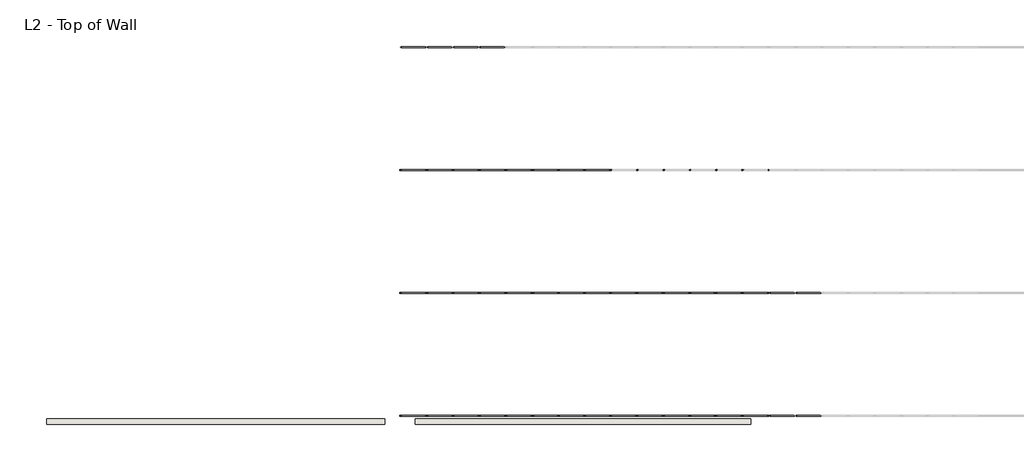
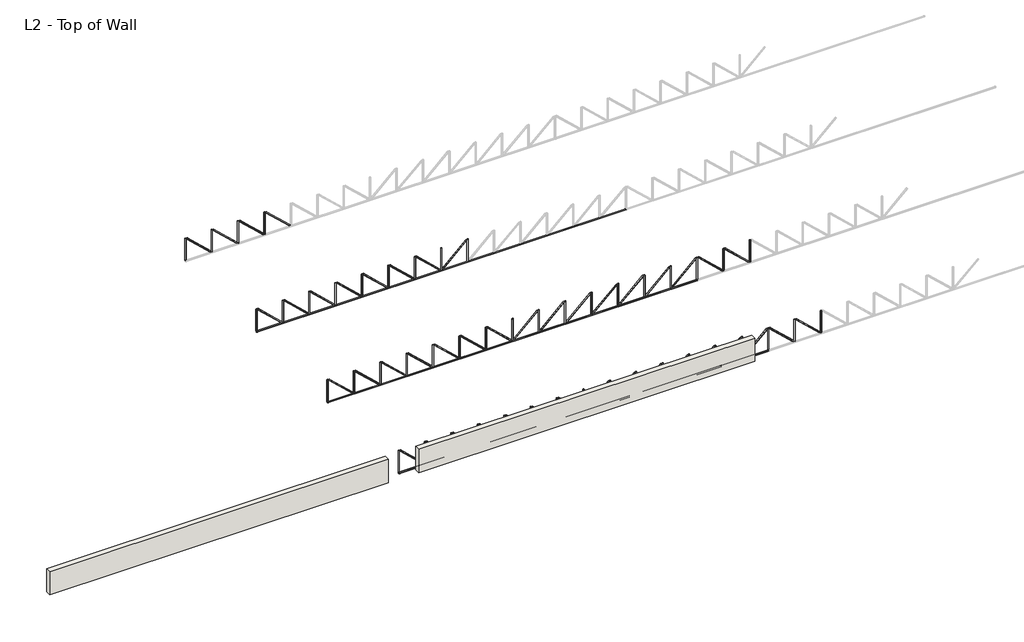
# One storey, part 1 of 4: 96 beams, 2 walls.
"""IFC4 building model written with IfcOpenShell, lengths in millimetres."""

import ifcopenshell
import ifcopenshell.guid

model = None  # the IFC model being written
_history = None  # IfcOwnerHistory: only IFC2X3 demands one
_inside = {}  # id of a spatial element -> (the spatial element, [elements in it])
_under = {}  # id of a project, library or spatial element -> (it, [spatial elements below it])
_declared = {}  # id of a project -> (the project, [libraries it declares])
_typed = {}  # id of a type object -> (the type object, [elements of that type])
_made_of = {}  # id of a material, layer set ... -> (it, [elements and type objects made of it])


def new_model(schema):
    """Start an empty IFC model of exactly this schema.

    Asked for "IFC4X3", IfcOpenShell would pick the latest addendum, in which some entities
    have other attributes; the version numbers below select the first issue.
    IFC2X3 requires an IfcOwnerHistory on every rooted entity: one is made here for all.
    """
    global model, _history
    if schema == "IFC4X3":
        model = ifcopenshell.file(schema_version=(4, 3, 0, 0))
    else:
        model = ifcopenshell.file(schema=schema)
    _inside.clear()
    _under.clear()
    _declared.clear()
    _typed.clear()
    _made_of.clear()
    _history = None
    if model.schema == "IFC2X3":
        org = make("IfcOrganization", Name="unknown")
        user = make(
            "IfcPersonAndOrganization",
            ThePerson=make("IfcPerson", FamilyName="unknown"),
            TheOrganization=org,
        )
        app = make(
            "IfcApplication",
            ApplicationDeveloper=org,
            Version="unknown",
            ApplicationFullName="unknown",
            ApplicationIdentifier="unknown",
        )
        _history = make(
            "IfcOwnerHistory",
            OwningUser=user,
            OwningApplication=app,
            ChangeAction="ADDED",
            CreationDate=0,
        )
    return model


def make(cls, **values):
    """One entity of the class cls with the attributes given. An attribute that is None is left unset."""
    return model.create_entity(
        cls, **{name: value for name, value in values.items() if value is not None}
    )


def rooted(cls, **values):
    """An entity with a GlobalId (a new one), such as an element, a storey or a relation."""
    return make(cls, GlobalId=ifcopenshell.guid.new(), OwnerHistory=_history, **values)


def si_unit(unit_type, name, prefix=None):
    """IfcSIUnit, for example si_unit("LENGTHUNIT", "METRE", prefix="MILLI")."""
    return make("IfcSIUnit", UnitType=unit_type, Prefix=prefix, Name=name)


def assignment(units):
    """IfcUnitAssignment: the units of a project."""
    return None if units is None else make("IfcUnitAssignment", Units=units)


def point(xyz):
    """IfcCartesianPoint."""
    return None if xyz is None else make("IfcCartesianPoint", Coordinates=xyz)


def direction(xyz):
    """IfcDirection."""
    return None if xyz is None else make("IfcDirection", DirectionRatios=xyz)


def frame(location, z_axis=None, x_axis=None):
    """IfcAxis2Placement3D, a coordinate frame: its origin and axes. An axis left out is left unset."""
    return make(
        "IfcAxis2Placement3D",
        Location=point(location),
        Axis=direction(z_axis),
        RefDirection=direction(x_axis),
    )


def frame_2d(location, x_axis=None):
    """IfcAxis2Placement2D, a coordinate frame in the plane: its origin and x axis."""
    return make(
        "IfcAxis2Placement2D", Location=point(location), RefDirection=direction(x_axis)
    )


def origin():
    """The frame at (0, 0, 0) with its axes left unset."""
    return frame((0.0, 0.0, 0.0))


def origin_2d():
    """The frame at (0, 0) in the plane with its x axis left unset."""
    return frame_2d((0.0, 0.0))


def place(relative_to, where):
    """IfcLocalPlacement: puts the frame where relative to a parent placement (None: the world)."""
    return make(
        "IfcLocalPlacement", PlacementRelTo=relative_to, RelativePlacement=where
    )


def context(
    kind, dimensions, precision=None, world=None, true_north=None, identifier=None
):
    """IfcGeometricRepresentationContext, for example the 3D "Model" context."""
    return make(
        "IfcGeometricRepresentationContext",
        ContextIdentifier=identifier,
        ContextType=kind,
        CoordinateSpaceDimension=dimensions,
        Precision=precision,
        WorldCoordinateSystem=world,
        TrueNorth=true_north,
    )


def project(units=None, contexts=None):
    """IfcProject with its units and contexts."""
    return rooted(
        "IfcProject",
        Name="project",
        RepresentationContexts=contexts,
        UnitsInContext=assignment(units),
    )


def spatial(cls, under=None, at=None, **own):
    """A site, building, storey or space (cls), placed at a placement, below another one or the project."""
    s = rooted(cls, ObjectPlacement=at, **own)
    if under is not None:
        _under.setdefault(under.id(), (under, []))[1].append(s)
    return s


def circle_curve(where, radius):
    """IfcCircle in the frame where."""
    return make("IfcCircle", Position=where, Radius=radius)


def trimmed(basis, trim1, trim2, sense, master):
    """IfcTrimmedCurve: the piece of a basis curve between two trims."""
    return make(
        "IfcTrimmedCurve",
        BasisCurve=basis,
        Trim1=trim1,
        Trim2=trim2,
        SenseAgreement=sense,
        MasterRepresentation=master,
    )


def segment(curve, same_sense, transition):
    """IfcCompositeCurveSegment."""
    return make(
        "IfcCompositeCurveSegment",
        Transition=transition,
        SameSense=same_sense,
        ParentCurve=curve,
    )


def composite_curve(segments, self_intersect=None):
    """IfcCompositeCurve: segments joined end to end."""
    return make("IfcCompositeCurve", Segments=segments, SelfIntersect=self_intersect)


def outline(outer, holes=None, kind="AREA"):
    """IfcArbitraryClosedProfileDef: a profile drawn as a closed curve; with holes, ...WithVoids."""
    if holes is None:
        return make("IfcArbitraryClosedProfileDef", ProfileType=kind, OuterCurve=outer)
    return make(
        "IfcArbitraryProfileDefWithVoids",
        ProfileType=kind,
        OuterCurve=outer,
        InnerCurves=holes,
    )


def extrude(swept, where, along, depth):
    """IfcExtrudedAreaSolid: the profile swept, set in the frame where, extruded along a direction by depth."""
    return make(
        "IfcExtrudedAreaSolid",
        SweptArea=swept,
        Position=where,
        ExtrudedDirection=direction(along),
        Depth=depth,
    )


def faces_of(points, faces, orient=None, outer=None):
    """IfcFace entities. A face is a list of loops; a loop is a list of indices into points, from 0.

    orient and outer hold one flag for each loop. By default every Orientation is true, the
    first loop of a face is its IfcFaceOuterBound and the others are IfcFaceBound.
    """
    made = []
    for i, loops in enumerate(faces):
        bounds = []
        for j, loop in enumerate(loops):
            is_outer = j == 0 if outer is None else outer[i][j]
            bounds.append(
                make(
                    "IfcFaceOuterBound" if is_outer else "IfcFaceBound",
                    Bound=make("IfcPolyLoop", Polygon=[points[k] for k in loop]),
                    Orientation=True if orient is None else orient[i][j],
                )
            )
        made.append(make("IfcFace", Bounds=bounds))
    return made


def faceted_brep(points, faces, orient=None, outer=None, voids=None):
    """IfcFacetedBrep: a solid bounded by flat faces; with voids (closed shells), ...WithVoids."""
    shared = [point(p) for p in points]
    hull = make("IfcClosedShell", CfsFaces=faces_of(shared, faces, orient, outer))
    if voids is None:
        return make("IfcFacetedBrep", Outer=hull)
    return make(
        "IfcFacetedBrepWithVoids",
        Outer=hull,
        Voids=[
            make(cls, CfsFaces=faces_of(shared, fs, o, b)) for cls, fs, o, b in voids
        ],
    )


def shape(context_of_items, identifier, shape_type, items):
    """IfcShapeRepresentation: the items that make up one representation, for example the "Body"."""
    return make(
        "IfcShapeRepresentation",
        ContextOfItems=context_of_items,
        RepresentationIdentifier=identifier,
        RepresentationType=shape_type,
        Items=items,
    )


def source(mapping_origin, context_of_items, identifier, shape_type, items):
    """IfcRepresentationMap: a shape defined once, which mapped items show again and again."""
    return make(
        "IfcRepresentationMap",
        MappingOrigin=mapping_origin,
        MappedRepresentation=shape(context_of_items, identifier, shape_type, items),
    )


def transform(
    local_origin,
    x_axis=None,
    y_axis=None,
    z_axis=None,
    scale=None,
    scale2=None,
    scale3=None,
    uniform=True,
):
    """IfcCartesianTransformationOperator3D, or its non-uniform kind. x_axis, y_axis, z_axis: its Axis1, 2, 3."""
    if uniform:
        return make(
            "IfcCartesianTransformationOperator3D",
            Axis1=direction(x_axis),
            Axis2=direction(y_axis),
            LocalOrigin=point(local_origin),
            Scale=scale,
            Axis3=direction(z_axis),
        )
    return make(
        "IfcCartesianTransformationOperator3DnonUniform",
        Axis1=direction(x_axis),
        Axis2=direction(y_axis),
        LocalOrigin=point(local_origin),
        Scale=scale,
        Axis3=direction(z_axis),
        Scale2=scale2,
        Scale3=scale3,
    )


def mapped(mapping_source, mapping_target):
    """IfcMappedItem: shows the shape of a source again, moved by a transform."""
    return make(
        "IfcMappedItem", MappingSource=mapping_source, MappingTarget=mapping_target
    )


def made_of(thing, what):
    """Note that an element or type object is made of a material, layer set ...; save() writes the relation."""
    if what is not None:
        _made_of.setdefault(what.id(), (what, []))[1].append(thing)
    return thing


def element(
    cls,
    number,
    at=None,
    inside=None,
    cuts=None,
    type_object=None,
    material=None,
    context=None,
    identifier="Body",
    shape_type=None,
    held_by="IfcProductDefinitionShape",
    body=None,
    shapes=None,
    **own,
):
    """One element of the class cls, such as IfcWall. Its Tag is "e" and its number.

    at: its placement. inside: the storey or other place that contains it. cuts: it is an
    opening in that element (IfcRelVoidsElement). A single representation is given by context,
    identifier, shape_type and body (its items); several are given by shapes. held_by: the class
    of the entity that holds the representations. save() writes the other relations.
    """
    e = rooted(cls, Tag="e%d" % number, ObjectPlacement=at, **own)
    if body is not None:
        shapes = [shape(context, identifier, shape_type, body)]
    if shapes is not None:
        e.Representation = make(held_by, Representations=shapes)
    if inside is not None:
        _inside.setdefault(inside.id(), (inside, []))[1].append(e)
    if cuts is not None:
        rooted(
            "IfcRelVoidsElement", RelatingBuildingElement=cuts, RelatedOpeningElement=e
        )
    if type_object is not None:
        _typed.setdefault(type_object.id(), (type_object, []))[1].append(e)
    return made_of(e, material)


def aggregate(whole, parts):
    """IfcRelAggregates: a whole, such as a stair, and the parts it consists of."""
    return rooted("IfcRelAggregates", RelatingObject=whole, RelatedObjects=parts)


def save(model, path):
    """Write the relations noted so far, then the file.

    IfcRelAggregates (storeys below a building ...), IfcRelContainedInSpatialStructure (elements
    in a storey), IfcRelDefinesByType, IfcRelAssociatesMaterial and IfcRelDeclares: one each for
    every whole, place, type object, material and project.
    """
    for whole, parts in _under.values():
        aggregate(whole, parts)
    for where, things in _inside.values():
        rooted(
            "IfcRelContainedInSpatialStructure",
            RelatedElements=things,
            RelatingStructure=where,
        )
    for kind, things in _typed.values():
        rooted("IfcRelDefinesByType", RelatedObjects=things, RelatingType=kind)
    for what, things in _made_of.values():
        rooted("IfcRelAssociatesMaterial", RelatedObjects=things, RelatingMaterial=what)
    for by, libraries in _declared.values():
        rooted("IfcRelDeclares", RelatingContext=by, RelatedDefinitions=libraries)
    model.write(path)


def circular_hollow_sections_chs60_3x5_c94bd862(model_context):
    return source(origin(), model_context, "Body", "SweptSolid", [
        extrude(outline(composite_curve([segment(trimmed(circle_curve(origin_2d(), 30.15), [point((-30.15, 0.0))], [point((30.15, 0.0))], False, "CARTESIAN"), True, "CONTINUOUS"), segment(trimmed(circle_curve(origin_2d(), 30.15), [point((30.15, 0.0))], [point((-30.15, 0.0))], False, "CARTESIAN"), True, "CONTINUOUS")], self_intersect=False), holes=[composite_curve([segment(trimmed(circle_curve(origin_2d(), 25.15), [point((25.15, 0.0))], [point((-25.15, 0.0))], True, "CARTESIAN"), True, "CONTINUOUS"), segment(trimmed(circle_curve(origin_2d(), 25.15), [point((-25.15, 0.0))], [point((25.15, 0.0))], True, "CARTESIAN"), True, "CONTINUOUS")], self_intersect=False)]), frame((-557.0, 0.0, 0.0), z_axis=(1.0, 0.0, 0.0), x_axis=(0.0, 1.0, 0.0)), (0.0, 0.0, 1.0), 1114.0),
    ])


def circular_hollow_sections_chs60_3x5_b8a643cb(model_context):
    return source(origin(), model_context, "Body", "SweptSolid", [
        extrude(outline(composite_curve([segment(trimmed(circle_curve(origin_2d(), 30.15), [point((-30.15, 0.0))], [point((30.15, 0.0))], False, "CARTESIAN"), True, "CONTINUOUS"), segment(trimmed(circle_curve(origin_2d(), 30.15), [point((30.15, 0.0))], [point((-30.15, 0.0))], False, "CARTESIAN"), True, "CONTINUOUS")], self_intersect=False), holes=[composite_curve([segment(trimmed(circle_curve(origin_2d(), 25.15), [point((25.15, 0.0))], [point((-25.15, 0.0))], True, "CARTESIAN"), True, "CONTINUOUS"), segment(trimmed(circle_curve(origin_2d(), 25.15), [point((-25.15, 0.0))], [point((25.15, 0.0))], True, "CARTESIAN"), True, "CONTINUOUS")], self_intersect=False)]), frame((-790.0, 0.0, 0.0), z_axis=(1.0, 0.0, 0.0), x_axis=(0.0, 1.0, 0.0)), (0.0, 0.0, 1.0), 1580.0),
    ])


def circular_hollow_sections_chs60_3x5_ee2473de(model_context):
    return source(origin(), model_context, "Body", "SweptSolid", [
        extrude(outline(composite_curve([segment(trimmed(circle_curve(origin_2d(), 30.15), [point((-30.15, 0.0))], [point((30.15, 0.0))], False, "CARTESIAN"), True, "CONTINUOUS"), segment(trimmed(circle_curve(origin_2d(), 30.15), [point((30.15, 0.0))], [point((-30.15, 0.0))], False, "CARTESIAN"), True, "CONTINUOUS")], self_intersect=False), holes=[composite_curve([segment(trimmed(circle_curve(origin_2d(), 25.15), [point((25.15, 0.0))], [point((-25.15, 0.0))], True, "CARTESIAN"), True, "CONTINUOUS"), segment(trimmed(circle_curve(origin_2d(), 25.15), [point((-25.15, 0.0))], [point((25.15, 0.0))], True, "CARTESIAN"), True, "CONTINUOUS")], self_intersect=False)]), frame((-9000.0, 0.0, 0.0), z_axis=(1.0, 0.0, 0.0), x_axis=(0.0, 1.0, 0.0)), (0.0, 0.0, 1.0), 18000.0),
    ])


model = new_model("IFC4")

# Units and contexts
model_context = context("Model", 3, world=origin())
ifc_project = project(units=[si_unit("LENGTHUNIT", "METRE", prefix="MILLI")], contexts=[model_context])

# Site, building, storey
site = spatial("IfcSite", under=ifc_project)
building = spatial("IfcBuilding", under=site)
storey = spatial("IfcBuildingStorey", under=building, Name="L2 - Top of Wall", Elevation=6600.0)

# Beams
placement = place(None, origin())
circular_hollow_sections_chs60_3x5_shape = circular_hollow_sections_chs60_3x5_c94bd862(model_context)
element("IfcBeam", 1, ObjectType="Circular Hollow Sections : CHS60.3x5", at=placement, inside=storey, context=model_context, shape_type="MappedRepresentation", body=[
    mapped(circular_hollow_sections_chs60_3x5_shape, transform((12147.60894, -5058.7619082, 7200.0), x_axis=(0.0, 0.0, 1.0), y_axis=(0.0, -1.0, 0.0), z_axis=(1.0, 0.0, 0.0))),
])
element("IfcBeam", 2, ObjectType="Circular Hollow Sections : CHS60.3x5", at=placement, inside=storey, context=model_context, shape_type="MappedRepresentation", body=[
    mapped(circular_hollow_sections_chs60_3x5_shape, transform((13433.3232257, -5058.7619082, 7200.0), x_axis=(0.0, 0.0, 1.0), y_axis=(0.0, -1.0, 0.0), z_axis=(1.0, 0.0, 0.0))),
])
element("IfcBeam", 3, ObjectType="Circular Hollow Sections : CHS60.3x5", at=placement, inside=storey, context=model_context, shape_type="MappedRepresentation", body=[
    mapped(circular_hollow_sections_chs60_3x5_shape, transform((14719.0375115, -5058.7619082, 7200.0), x_axis=(0.0, 0.0, 1.0), y_axis=(0.0, -1.0, 0.0), z_axis=(1.0, 0.0, 0.0))),
])
element("IfcBeam", 4, ObjectType="Circular Hollow Sections : CHS60.3x5", at=placement, inside=storey, context=model_context, shape_type="MappedRepresentation", body=[
    mapped(circular_hollow_sections_chs60_3x5_shape, transform((10861.8946543, -5058.7619082, 7200.0), x_axis=(0.0, 0.0, 1.0), y_axis=(0.0, -1.0, 0.0), z_axis=(1.0, 0.0, 0.0))),
])
element("IfcBeam", 5, ObjectType="Circular Hollow Sections : CHS60.3x5", at=placement, inside=storey, context=model_context, shape_type="MappedRepresentation", body=[
    mapped(circular_hollow_sections_chs60_3x5_shape, transform((12146.15894, -11058.7619082, 7200.0), x_axis=(0.0, 0.0, 1.0), y_axis=(0.0, -1.0, 0.0), z_axis=(1.0, 0.0, 0.0))),
])
element("IfcBeam", 6, ObjectType="Circular Hollow Sections : CHS60.3x5", at=placement, inside=storey, context=model_context, shape_type="MappedRepresentation", body=[
    mapped(circular_hollow_sections_chs60_3x5_shape, transform((13431.8732257, -11058.7619082, 7200.0), x_axis=(0.0, 0.0, 1.0), y_axis=(0.0, -1.0, 0.0), z_axis=(1.0, 0.0, 0.0))),
])
element("IfcBeam", 7, ObjectType="Circular Hollow Sections : CHS60.3x5", at=placement, inside=storey, context=model_context, shape_type="MappedRepresentation", body=[
    mapped(circular_hollow_sections_chs60_3x5_shape, transform((14717.5875115, -11058.7619082, 7200.0), x_axis=(0.0, 0.0, 1.0), y_axis=(0.0, -1.0, 0.0), z_axis=(1.0, 0.0, 0.0))),
])
element("IfcBeam", 8, ObjectType="Circular Hollow Sections : CHS60.3x5", at=placement, inside=storey, context=model_context, shape_type="MappedRepresentation", body=[
    mapped(circular_hollow_sections_chs60_3x5_shape, transform((21146.15894, -11058.7619082, 7200.0), x_axis=(0.0, 0.0, 1.0), y_axis=(0.0, -1.0, 0.0), z_axis=(1.0, 0.0, 0.0))),
])
element("IfcBeam", 9, ObjectType="Circular Hollow Sections : CHS60.3x5", at=placement, inside=storey, context=model_context, shape_type="MappedRepresentation", body=[
    mapped(circular_hollow_sections_chs60_3x5_shape, transform((16003.3017972, -11058.7619082, 7200.0), x_axis=(0.0, 0.0, 1.0), y_axis=(0.0, -1.0, 0.0), z_axis=(1.0, 0.0, 0.0))),
])
element("IfcBeam", 10, ObjectType="Circular Hollow Sections : CHS60.3x5", at=placement, inside=storey, context=model_context, shape_type="MappedRepresentation", body=[
    mapped(circular_hollow_sections_chs60_3x5_shape, transform((17289.0160829, -11058.7619082, 7200.0), x_axis=(0.0, 0.0, 1.0), y_axis=(0.0, -1.0, 0.0), z_axis=(1.0, 0.0, 0.0))),
])
element("IfcBeam", 11, ObjectType="Circular Hollow Sections : CHS60.3x5", at=placement, inside=storey, context=model_context, shape_type="MappedRepresentation", body=[
    mapped(circular_hollow_sections_chs60_3x5_shape, transform((10860.4446543, -11058.7619082, 7200.0), x_axis=(0.0, 0.0, 1.0), y_axis=(0.0, -1.0, 0.0), z_axis=(1.0, 0.0, 0.0))),
])
element("IfcBeam", 12, ObjectType="Circular Hollow Sections : CHS60.3x5", at=placement, inside=storey, context=model_context, shape_type="MappedRepresentation", body=[
    mapped(circular_hollow_sections_chs60_3x5_shape, transform((18574.7303686, -11058.7619082, 7200.0), x_axis=(0.0, 0.0, 1.0), y_axis=(0.0, -1.0, 0.0), z_axis=(1.0, 0.0, 0.0))),
])
element("IfcBeam", 13, ObjectType="Circular Hollow Sections : CHS60.3x5", at=placement, inside=storey, context=model_context, shape_type="MappedRepresentation", body=[
    mapped(circular_hollow_sections_chs60_3x5_shape, transform((19860.4446543, -11058.7619082, 7200.0), x_axis=(0.0, 0.0, 1.0), y_axis=(0.0, -1.0, 0.0), z_axis=(1.0, 0.0, 0.0))),
])
element("IfcBeam", 14, ObjectType="Circular Hollow Sections : CHS60.3x5", at=placement, inside=storey, context=model_context, shape_type="MappedRepresentation", body=[
    mapped(circular_hollow_sections_chs60_3x5_shape, transform((27574.7303686, -17058.7619082, 7200.0), x_axis=(0.0, 0.0, 1.0), y_axis=(0.0, -1.0, 0.0), z_axis=(1.0, 0.0, 0.0))),
])
element("IfcBeam", 15, ObjectType="Circular Hollow Sections : CHS60.3x5", at=placement, inside=storey, context=model_context, shape_type="MappedRepresentation", body=[
    mapped(circular_hollow_sections_chs60_3x5_shape, transform((12146.15894, -17058.7619082, 7200.0), x_axis=(0.0, 0.0, 1.0), y_axis=(0.0, -1.0, 0.0), z_axis=(1.0, 0.0, 0.0))),
])
element("IfcBeam", 16, ObjectType="Circular Hollow Sections : CHS60.3x5", at=placement, inside=storey, context=model_context, shape_type="MappedRepresentation", body=[
    mapped(circular_hollow_sections_chs60_3x5_shape, transform((26289.0160829, -17058.7619082, 7200.0), x_axis=(0.0, 0.0, 1.0), y_axis=(0.0, -1.0, 0.0), z_axis=(1.0, 0.0, 0.0))),
])
element("IfcBeam", 17, ObjectType="Circular Hollow Sections : CHS60.3x5", at=placement, inside=storey, context=model_context, shape_type="MappedRepresentation", body=[
    mapped(circular_hollow_sections_chs60_3x5_shape, transform((13431.8732257, -17058.7619082, 7200.0), x_axis=(0.0, 0.0, 1.0), y_axis=(0.0, -1.0, 0.0), z_axis=(1.0, 0.0, 0.0))),
])
element("IfcBeam", 18, ObjectType="Circular Hollow Sections : CHS60.3x5", at=placement, inside=storey, context=model_context, shape_type="MappedRepresentation", body=[
    mapped(circular_hollow_sections_chs60_3x5_shape, transform((25003.3017972, -17058.7619082, 7200.0), x_axis=(0.0, 0.0, 1.0), y_axis=(0.0, -1.0, 0.0), z_axis=(1.0, 0.0, 0.0))),
])
element("IfcBeam", 19, ObjectType="Circular Hollow Sections : CHS60.3x5", at=placement, inside=storey, context=model_context, shape_type="MappedRepresentation", body=[
    mapped(circular_hollow_sections_chs60_3x5_shape, transform((14717.5875115, -17058.7619082, 7200.0), x_axis=(0.0, 0.0, 1.0), y_axis=(0.0, -1.0, 0.0), z_axis=(1.0, 0.0, 0.0))),
])
element("IfcBeam", 20, ObjectType="Circular Hollow Sections : CHS60.3x5", at=placement, inside=storey, context=model_context, shape_type="MappedRepresentation", body=[
    mapped(circular_hollow_sections_chs60_3x5_shape, transform((23717.5875115, -17058.7619082, 7200.0), x_axis=(0.0, 0.0, 1.0), y_axis=(0.0, -1.0, 0.0), z_axis=(1.0, 0.0, 0.0))),
])
element("IfcBeam", 21, ObjectType="Circular Hollow Sections : CHS60.3x5", at=placement, inside=storey, context=model_context, shape_type="MappedRepresentation", body=[
    mapped(circular_hollow_sections_chs60_3x5_shape, transform((22431.8732257, -17058.7619082, 7200.0), x_axis=(0.0, 0.0, 1.0), y_axis=(0.0, -1.0, 0.0), z_axis=(1.0, 0.0, 0.0))),
])
element("IfcBeam", 22, ObjectType="Circular Hollow Sections : CHS60.3x5", at=placement, inside=storey, context=model_context, shape_type="MappedRepresentation", body=[
    mapped(circular_hollow_sections_chs60_3x5_shape, transform((28860.4446543, -17058.7619082, 7200.0), x_axis=(0.0, 0.0, 1.0), y_axis=(0.0, -1.0, 0.0), z_axis=(1.0, 0.0, 0.0))),
])
element("IfcBeam", 23, ObjectType="Circular Hollow Sections : CHS60.3x5", at=placement, inside=storey, context=model_context, shape_type="MappedRepresentation", body=[
    mapped(circular_hollow_sections_chs60_3x5_shape, transform((21146.15894, -17058.7619082, 7200.0), x_axis=(0.0, 0.0, 1.0), y_axis=(0.0, -1.0, 0.0), z_axis=(1.0, 0.0, 0.0))),
])
element("IfcBeam", 24, ObjectType="Circular Hollow Sections : CHS60.3x5", at=placement, inside=storey, context=model_context, shape_type="MappedRepresentation", body=[
    mapped(circular_hollow_sections_chs60_3x5_shape, transform((16003.3017972, -17058.7619082, 7200.0), x_axis=(0.0, 0.0, 1.0), y_axis=(0.0, -1.0, 0.0), z_axis=(1.0, 0.0, 0.0))),
])
element("IfcBeam", 25, ObjectType="Circular Hollow Sections : CHS60.3x5", at=placement, inside=storey, context=model_context, shape_type="MappedRepresentation", body=[
    mapped(circular_hollow_sections_chs60_3x5_shape, transform((17289.0160829, -17058.7619082, 7200.0), x_axis=(0.0, 0.0, 1.0), y_axis=(0.0, -1.0, 0.0), z_axis=(1.0, 0.0, 0.0))),
])
element("IfcBeam", 26, ObjectType="Circular Hollow Sections : CHS60.3x5", at=placement, inside=storey, context=model_context, shape_type="MappedRepresentation", body=[
    mapped(circular_hollow_sections_chs60_3x5_shape, transform((10860.4446543, -17058.7619082, 7200.0), x_axis=(0.0, 0.0, 1.0), y_axis=(0.0, -1.0, 0.0), z_axis=(1.0, 0.0, 0.0))),
])
element("IfcBeam", 27, ObjectType="Circular Hollow Sections : CHS60.3x5", at=placement, inside=storey, context=model_context, shape_type="MappedRepresentation", body=[
    mapped(circular_hollow_sections_chs60_3x5_shape, transform((18574.7303686, -17058.7619082, 7200.0), x_axis=(0.0, 0.0, 1.0), y_axis=(0.0, -1.0, 0.0), z_axis=(1.0, 0.0, 0.0))),
])
element("IfcBeam", 28, ObjectType="Circular Hollow Sections : CHS60.3x5", at=placement, inside=storey, context=model_context, shape_type="MappedRepresentation", body=[
    mapped(circular_hollow_sections_chs60_3x5_shape, transform((19860.4446543, -17058.7619082, 7200.0), x_axis=(0.0, 0.0, 1.0), y_axis=(0.0, -1.0, 0.0), z_axis=(1.0, 0.0, 0.0))),
])
element("IfcBeam", 29, ObjectType="Circular Hollow Sections : CHS60.3x5", at=placement, inside=storey, context=model_context, shape_type="MappedRepresentation", body=[
    mapped(circular_hollow_sections_chs60_3x5_shape, transform((27574.7303686, -23058.7619082, 7200.0), x_axis=(0.0, 0.0, 1.0), y_axis=(0.0, -1.0, 0.0), z_axis=(1.0, 0.0, 0.0))),
])
element("IfcBeam", 30, ObjectType="Circular Hollow Sections : CHS60.3x5", at=placement, inside=storey, context=model_context, shape_type="MappedRepresentation", body=[
    mapped(circular_hollow_sections_chs60_3x5_shape, transform((12146.15894, -23058.7619082, 7200.0), x_axis=(0.0, 0.0, 1.0), y_axis=(0.0, -1.0, 0.0), z_axis=(1.0, 0.0, 0.0))),
])
element("IfcBeam", 31, ObjectType="Circular Hollow Sections : CHS60.3x5", at=placement, inside=storey, context=model_context, shape_type="MappedRepresentation", body=[
    mapped(circular_hollow_sections_chs60_3x5_shape, transform((26289.0160829, -23058.7619082, 7200.0), x_axis=(0.0, 0.0, 1.0), y_axis=(0.0, -1.0, 0.0), z_axis=(1.0, 0.0, 0.0))),
])
element("IfcBeam", 32, ObjectType="Circular Hollow Sections : CHS60.3x5", at=placement, inside=storey, context=model_context, shape_type="MappedRepresentation", body=[
    mapped(circular_hollow_sections_chs60_3x5_shape, transform((13431.8732257, -23058.7619082, 7200.0), x_axis=(0.0, 0.0, 1.0), y_axis=(0.0, -1.0, 0.0), z_axis=(1.0, 0.0, 0.0))),
])
element("IfcBeam", 33, ObjectType="Circular Hollow Sections : CHS60.3x5", at=placement, inside=storey, context=model_context, shape_type="MappedRepresentation", body=[
    mapped(circular_hollow_sections_chs60_3x5_shape, transform((25003.3017972, -23058.7619082, 7200.0), x_axis=(0.0, 0.0, 1.0), y_axis=(0.0, -1.0, 0.0), z_axis=(1.0, 0.0, 0.0))),
])
element("IfcBeam", 34, ObjectType="Circular Hollow Sections : CHS60.3x5", at=placement, inside=storey, context=model_context, shape_type="MappedRepresentation", body=[
    mapped(circular_hollow_sections_chs60_3x5_shape, transform((14717.5875115, -23058.7619082, 7200.0), x_axis=(0.0, 0.0, 1.0), y_axis=(0.0, -1.0, 0.0), z_axis=(1.0, 0.0, 0.0))),
])
element("IfcBeam", 35, ObjectType="Circular Hollow Sections : CHS60.3x5", at=placement, inside=storey, context=model_context, shape_type="MappedRepresentation", body=[
    mapped(circular_hollow_sections_chs60_3x5_shape, transform((23717.5875115, -23058.7619082, 7200.0), x_axis=(0.0, 0.0, 1.0), y_axis=(0.0, -1.0, 0.0), z_axis=(1.0, 0.0, 0.0))),
])
element("IfcBeam", 36, ObjectType="Circular Hollow Sections : CHS60.3x5", at=placement, inside=storey, context=model_context, shape_type="MappedRepresentation", body=[
    mapped(circular_hollow_sections_chs60_3x5_shape, transform((22431.8732257, -23058.7619082, 7200.0), x_axis=(0.0, 0.0, 1.0), y_axis=(0.0, -1.0, 0.0), z_axis=(1.0, 0.0, 0.0))),
])
element("IfcBeam", 37, ObjectType="Circular Hollow Sections : CHS60.3x5", at=placement, inside=storey, context=model_context, shape_type="MappedRepresentation", body=[
    mapped(circular_hollow_sections_chs60_3x5_shape, transform((28860.4446543, -23058.7619082, 7200.0), x_axis=(0.0, 0.0, 1.0), y_axis=(0.0, -1.0, 0.0), z_axis=(1.0, 0.0, 0.0))),
])
element("IfcBeam", 38, ObjectType="Circular Hollow Sections : CHS60.3x5", at=placement, inside=storey, context=model_context, shape_type="MappedRepresentation", body=[
    mapped(circular_hollow_sections_chs60_3x5_shape, transform((21146.15894, -23058.7619082, 7200.0), x_axis=(0.0, 0.0, 1.0), y_axis=(0.0, -1.0, 0.0), z_axis=(1.0, 0.0, 0.0))),
])
element("IfcBeam", 39, ObjectType="Circular Hollow Sections : CHS60.3x5", at=placement, inside=storey, context=model_context, shape_type="MappedRepresentation", body=[
    mapped(circular_hollow_sections_chs60_3x5_shape, transform((16003.3017972, -23058.7619082, 7200.0), x_axis=(0.0, 0.0, 1.0), y_axis=(0.0, -1.0, 0.0), z_axis=(1.0, 0.0, 0.0))),
])
element("IfcBeam", 40, ObjectType="Circular Hollow Sections : CHS60.3x5", at=placement, inside=storey, context=model_context, shape_type="MappedRepresentation", body=[
    mapped(circular_hollow_sections_chs60_3x5_shape, transform((17289.0160829, -23058.7619082, 7200.0), x_axis=(0.0, 0.0, 1.0), y_axis=(0.0, -1.0, 0.0), z_axis=(1.0, 0.0, 0.0))),
])
element("IfcBeam", 41, ObjectType="Circular Hollow Sections : CHS60.3x5", at=placement, inside=storey, context=model_context, shape_type="MappedRepresentation", body=[
    mapped(circular_hollow_sections_chs60_3x5_shape, transform((10860.4446543, -23058.7619082, 7200.0), x_axis=(0.0, 0.0, 1.0), y_axis=(0.0, -1.0, 0.0), z_axis=(1.0, 0.0, 0.0))),
])
element("IfcBeam", 42, ObjectType="Circular Hollow Sections : CHS60.3x5", at=placement, inside=storey, context=model_context, shape_type="MappedRepresentation", body=[
    mapped(circular_hollow_sections_chs60_3x5_shape, transform((18574.7303686, -23058.7619082, 7200.0), x_axis=(0.0, 0.0, 1.0), y_axis=(0.0, -1.0, 0.0), z_axis=(1.0, 0.0, 0.0))),
])
element("IfcBeam", 43, ObjectType="Circular Hollow Sections : CHS60.3x5", at=placement, inside=storey, context=model_context, shape_type="MappedRepresentation", body=[
    mapped(circular_hollow_sections_chs60_3x5_shape, transform((19860.4446543, -23058.7619082, 7200.0), x_axis=(0.0, 0.0, 1.0), y_axis=(0.0, -1.0, 0.0), z_axis=(1.0, 0.0, 0.0))),
])
element("IfcBeam", 44, ObjectType="Circular Hollow Sections : CHS60.3x5", at=placement, inside=storey, context=model_context, shape_type="MappedRepresentation", body=[
    mapped(circular_hollow_sections_chs60_3x5_shape, transform((30146.15894, -17058.7619082, 7200.0), x_axis=(0.0, 0.0, 1.0), y_axis=(0.0, -1.0, 0.0), z_axis=(1.0, 0.0, 0.0))),
])
element("IfcBeam", 45, ObjectType="Circular Hollow Sections : CHS60.3x5", at=placement, inside=storey, context=model_context, shape_type="MappedRepresentation", body=[
    mapped(circular_hollow_sections_chs60_3x5_shape, transform((31431.8732257, -17058.7619082, 7200.0), x_axis=(0.0, 0.0, 1.0), y_axis=(0.0, -1.0, 0.0), z_axis=(1.0, 0.0, 0.0))),
])
element("IfcBeam", 46, ObjectType="Circular Hollow Sections : CHS60.3x5", at=placement, inside=storey, context=model_context, shape_type="MappedRepresentation", body=[
    mapped(circular_hollow_sections_chs60_3x5_shape, transform((28860.4446543, -17058.7619082, 7200.0), x_axis=(0.0, 0.0, 1.0), y_axis=(0.0, -1.0, 0.0), z_axis=(1.0, 0.0, 0.0))),
])
element("IfcBeam", 47, ObjectType="Circular Hollow Sections : CHS60.3x5", at=placement, inside=storey, context=model_context, shape_type="MappedRepresentation", body=[
    mapped(circular_hollow_sections_chs60_3x5_shape, transform((30146.15894, -23058.7619082, 7200.0), x_axis=(0.0, 0.0, 1.0), y_axis=(0.0, -1.0, 0.0), z_axis=(1.0, 0.0, 0.0))),
])
element("IfcBeam", 48, ObjectType="Circular Hollow Sections : CHS60.3x5", at=placement, inside=storey, context=model_context, shape_type="MappedRepresentation", body=[
    mapped(circular_hollow_sections_chs60_3x5_shape, transform((31431.8732257, -23058.7619082, 7200.0), x_axis=(0.0, 0.0, 1.0), y_axis=(0.0, -1.0, 0.0), z_axis=(1.0, 0.0, 0.0))),
])
element("IfcBeam", 49, ObjectType="Circular Hollow Sections : CHS60.3x5", at=placement, inside=storey, context=model_context, shape_type="MappedRepresentation", body=[
    mapped(circular_hollow_sections_chs60_3x5_shape, transform((28860.4446543, -23058.7619082, 7200.0), x_axis=(0.0, 0.0, 1.0), y_axis=(0.0, -1.0, 0.0), z_axis=(1.0, 0.0, 0.0))),
])
circular_hollow_sections_chs60_3x5_2_shape = circular_hollow_sections_chs60_3x5_b8a643cb(model_context)
element("IfcBeam", 50, ObjectType="Circular Hollow Sections : CHS60.3x5", at=placement, inside=storey, context=model_context, shape_type="MappedRepresentation", body=[
    mapped(circular_hollow_sections_chs60_3x5_2_shape, transform((12790.4660829, -5058.7619082, 7200.0), x_axis=(0.7310552682428691, 0.0, -0.6823182503600111), y_axis=(0.0, -1.0, 0.0), z_axis=(-0.6823182503600111, 0.0, -0.7310552682428691))),
])
element("IfcBeam", 51, ObjectType="Circular Hollow Sections : CHS60.3x5", at=placement, inside=storey, context=model_context, shape_type="MappedRepresentation", body=[
    mapped(circular_hollow_sections_chs60_3x5_2_shape, transform((14076.1803686, -5058.7619082, 7200.0), x_axis=(0.7310552682428691, 0.0, -0.6823182503600111), y_axis=(0.0, -1.0, 0.0), z_axis=(-0.6823182503600111, 0.0, -0.7310552682428691))),
])
element("IfcBeam", 52, ObjectType="Circular Hollow Sections : CHS60.3x5", at=placement, inside=storey, context=model_context, shape_type="MappedRepresentation", body=[
    mapped(circular_hollow_sections_chs60_3x5_2_shape, transform((15361.8946543, -5058.7619082, 7200.0), x_axis=(0.7310552682428691, 0.0, -0.6823182503600111), y_axis=(0.0, -1.0, 0.0), z_axis=(-0.6823182503600111, 0.0, -0.7310552682428691))),
])
element("IfcBeam", 53, ObjectType="Circular Hollow Sections : CHS60.3x5", at=placement, inside=storey, context=model_context, shape_type="MappedRepresentation", body=[
    mapped(circular_hollow_sections_chs60_3x5_2_shape, transform((11504.7517972, -5058.7619082, 7200.0), x_axis=(0.7310552682428691, 0.0, -0.6823182503600111), y_axis=(0.0, -1.0, 0.0), z_axis=(-0.6823182503600111, 0.0, -0.7310552682428691))),
])
element("IfcBeam", 54, ObjectType="Circular Hollow Sections : CHS60.3x5", at=placement, inside=storey, context=model_context, shape_type="MappedRepresentation", body=[
    mapped(circular_hollow_sections_chs60_3x5_2_shape, transform((12789.0160829, -11058.7619082, 7200.0), x_axis=(0.7310552682428691, 0.0, -0.6823182503600111), y_axis=(0.0, -1.0, 0.0), z_axis=(-0.6823182503600111, 0.0, -0.7310552682428691))),
])
element("IfcBeam", 55, ObjectType="Circular Hollow Sections : CHS60.3x5", at=placement, inside=storey, context=model_context, shape_type="MappedRepresentation", body=[
    mapped(circular_hollow_sections_chs60_3x5_2_shape, transform((14074.7303686, -11058.7619082, 7200.0), x_axis=(0.7310552682428691, 0.0, -0.6823182503600111), y_axis=(0.0, -1.0, 0.0), z_axis=(-0.6823182503600111, 0.0, -0.7310552682428691))),
])
element("IfcBeam", 56, ObjectType="Circular Hollow Sections : CHS60.3x5", at=placement, inside=storey, context=model_context, shape_type="MappedRepresentation", body=[
    mapped(circular_hollow_sections_chs60_3x5_2_shape, transform((15360.4446543, -11058.7619082, 7200.0), x_axis=(0.7310552682428691, 0.0, -0.6823182503600111), y_axis=(0.0, -1.0, 0.0), z_axis=(-0.6823182503600111, 0.0, -0.7310552682428691))),
])
element("IfcBeam", 57, ObjectType="Circular Hollow Sections : CHS60.3x5", at=placement, inside=storey, context=model_context, shape_type="MappedRepresentation", body=[
    mapped(circular_hollow_sections_chs60_3x5_2_shape, transform((20503.3017972, -11058.7619082, 7200.0), x_axis=(0.7310552682428697, 0.0, 0.6823182503600105), y_axis=(0.0, -1.0, 0.0), z_axis=(0.6823182503600105, 0.0, -0.7310552682428697))),
])
element("IfcBeam", 58, ObjectType="Circular Hollow Sections : CHS60.3x5", at=placement, inside=storey, context=model_context, shape_type="MappedRepresentation", body=[
    mapped(circular_hollow_sections_chs60_3x5_2_shape, transform((16646.15894, -11058.7619082, 7200.0), x_axis=(0.7310552682428691, 0.0, -0.6823182503600111), y_axis=(0.0, -1.0, 0.0), z_axis=(-0.6823182503600111, 0.0, -0.7310552682428691))),
])
element("IfcBeam", 59, ObjectType="Circular Hollow Sections : CHS60.3x5", at=placement, inside=storey, context=model_context, shape_type="MappedRepresentation", body=[
    mapped(circular_hollow_sections_chs60_3x5_2_shape, transform((17931.8732257, -11058.7619082, 7200.0), x_axis=(0.7310552682428691, 0.0, -0.6823182503600111), y_axis=(0.0, -1.0, 0.0), z_axis=(-0.6823182503600111, 0.0, -0.7310552682428691))),
])
element("IfcBeam", 60, ObjectType="Circular Hollow Sections : CHS60.3x5", at=placement, inside=storey, context=model_context, shape_type="MappedRepresentation", body=[
    mapped(circular_hollow_sections_chs60_3x5_2_shape, transform((11503.3017972, -11058.7619082, 7200.0), x_axis=(0.7310552682428691, 0.0, -0.6823182503600111), y_axis=(0.0, -1.0, 0.0), z_axis=(-0.6823182503600111, 0.0, -0.7310552682428691))),
])
element("IfcBeam", 61, ObjectType="Circular Hollow Sections : CHS60.3x5", at=placement, inside=storey, context=model_context, shape_type="MappedRepresentation", body=[
    mapped(circular_hollow_sections_chs60_3x5_2_shape, transform((19217.5875115, -11058.7619082, 7200.0), x_axis=(0.7310552682428686, 0.0, -0.6823182503600118), y_axis=(0.0, -1.0, 0.0), z_axis=(-0.6823182503600118, 0.0, -0.7310552682428686))),
])
element("IfcBeam", 62, ObjectType="Circular Hollow Sections : CHS60.3x5", at=placement, inside=storey, context=model_context, shape_type="MappedRepresentation", body=[
    mapped(circular_hollow_sections_chs60_3x5_2_shape, transform((26931.8732257, -17058.7619082, 7200.0), x_axis=(0.7310552682428697, 0.0, 0.6823182503600105), y_axis=(0.0, -1.0, 0.0), z_axis=(0.6823182503600105, 0.0, -0.7310552682428697))),
])
element("IfcBeam", 63, ObjectType="Circular Hollow Sections : CHS60.3x5", at=placement, inside=storey, context=model_context, shape_type="MappedRepresentation", body=[
    mapped(circular_hollow_sections_chs60_3x5_2_shape, transform((12789.0160829, -17058.7619082, 7200.0), x_axis=(0.7310552682428691, 0.0, -0.6823182503600111), y_axis=(0.0, -1.0, 0.0), z_axis=(-0.6823182503600111, 0.0, -0.7310552682428691))),
])
element("IfcBeam", 64, ObjectType="Circular Hollow Sections : CHS60.3x5", at=placement, inside=storey, context=model_context, shape_type="MappedRepresentation", body=[
    mapped(circular_hollow_sections_chs60_3x5_2_shape, transform((25646.15894, -17058.7619082, 7200.0), x_axis=(0.7310552682428697, 0.0, 0.6823182503600105), y_axis=(0.0, -1.0, 0.0), z_axis=(0.6823182503600105, 0.0, -0.7310552682428697))),
])
element("IfcBeam", 65, ObjectType="Circular Hollow Sections : CHS60.3x5", at=placement, inside=storey, context=model_context, shape_type="MappedRepresentation", body=[
    mapped(circular_hollow_sections_chs60_3x5_2_shape, transform((14074.7303686, -17058.7619082, 7200.0), x_axis=(0.7310552682428691, 0.0, -0.6823182503600111), y_axis=(0.0, -1.0, 0.0), z_axis=(-0.6823182503600111, 0.0, -0.7310552682428691))),
])
element("IfcBeam", 66, ObjectType="Circular Hollow Sections : CHS60.3x5", at=placement, inside=storey, context=model_context, shape_type="MappedRepresentation", body=[
    mapped(circular_hollow_sections_chs60_3x5_2_shape, transform((24360.4446543, -17058.7619082, 7200.0), x_axis=(0.7310552682428697, 0.0, 0.6823182503600105), y_axis=(0.0, -1.0, 0.0), z_axis=(0.6823182503600105, 0.0, -0.7310552682428697))),
])
element("IfcBeam", 67, ObjectType="Circular Hollow Sections : CHS60.3x5", at=placement, inside=storey, context=model_context, shape_type="MappedRepresentation", body=[
    mapped(circular_hollow_sections_chs60_3x5_2_shape, transform((15360.4446543, -17058.7619082, 7200.0), x_axis=(0.7310552682428691, 0.0, -0.6823182503600111), y_axis=(0.0, -1.0, 0.0), z_axis=(-0.6823182503600111, 0.0, -0.7310552682428691))),
])
element("IfcBeam", 68, ObjectType="Circular Hollow Sections : CHS60.3x5", at=placement, inside=storey, context=model_context, shape_type="MappedRepresentation", body=[
    mapped(circular_hollow_sections_chs60_3x5_2_shape, transform((23074.7303686, -17058.7619082, 7200.0), x_axis=(0.7310552682428697, 0.0, 0.6823182503600105), y_axis=(0.0, -1.0, 0.0), z_axis=(0.6823182503600105, 0.0, -0.7310552682428697))),
])
element("IfcBeam", 69, ObjectType="Circular Hollow Sections : CHS60.3x5", at=placement, inside=storey, context=model_context, shape_type="MappedRepresentation", body=[
    mapped(circular_hollow_sections_chs60_3x5_2_shape, transform((21789.0160829, -17058.7619082, 7200.0), x_axis=(0.7310552682428697, 0.0, 0.6823182503600105), y_axis=(0.0, -1.0, 0.0), z_axis=(0.6823182503600105, 0.0, -0.7310552682428697))),
])
element("IfcBeam", 70, ObjectType="Circular Hollow Sections : CHS60.3x5", at=placement, inside=storey, context=model_context, shape_type="MappedRepresentation", body=[
    mapped(circular_hollow_sections_chs60_3x5_2_shape, transform((28217.5875115, -17058.7619082, 7200.0), x_axis=(0.7310552682428697, 0.0, 0.6823182503600105), y_axis=(0.0, -1.0, 0.0), z_axis=(0.6823182503600105, 0.0, -0.7310552682428697))),
])
element("IfcBeam", 71, ObjectType="Circular Hollow Sections : CHS60.3x5", at=placement, inside=storey, context=model_context, shape_type="MappedRepresentation", body=[
    mapped(circular_hollow_sections_chs60_3x5_2_shape, transform((20503.3017972, -17058.7619082, 7200.0), x_axis=(0.7310552682428697, 0.0, 0.6823182503600105), y_axis=(0.0, -1.0, 0.0), z_axis=(0.6823182503600105, 0.0, -0.7310552682428697))),
])
element("IfcBeam", 72, ObjectType="Circular Hollow Sections : CHS60.3x5", at=placement, inside=storey, context=model_context, shape_type="MappedRepresentation", body=[
    mapped(circular_hollow_sections_chs60_3x5_2_shape, transform((16646.15894, -17058.7619082, 7200.0), x_axis=(0.7310552682428691, 0.0, -0.6823182503600111), y_axis=(0.0, -1.0, 0.0), z_axis=(-0.6823182503600111, 0.0, -0.7310552682428691))),
])
element("IfcBeam", 73, ObjectType="Circular Hollow Sections : CHS60.3x5", at=placement, inside=storey, context=model_context, shape_type="MappedRepresentation", body=[
    mapped(circular_hollow_sections_chs60_3x5_2_shape, transform((17931.8732257, -17058.7619082, 7200.0), x_axis=(0.7310552682428691, 0.0, -0.6823182503600111), y_axis=(0.0, -1.0, 0.0), z_axis=(-0.6823182503600111, 0.0, -0.7310552682428691))),
])
element("IfcBeam", 74, ObjectType="Circular Hollow Sections : CHS60.3x5", at=placement, inside=storey, context=model_context, shape_type="MappedRepresentation", body=[
    mapped(circular_hollow_sections_chs60_3x5_2_shape, transform((11503.3017972, -17058.7619082, 7200.0), x_axis=(0.7310552682428691, 0.0, -0.6823182503600111), y_axis=(0.0, -1.0, 0.0), z_axis=(-0.6823182503600111, 0.0, -0.7310552682428691))),
])
element("IfcBeam", 75, ObjectType="Circular Hollow Sections : CHS60.3x5", at=placement, inside=storey, context=model_context, shape_type="MappedRepresentation", body=[
    mapped(circular_hollow_sections_chs60_3x5_2_shape, transform((19217.5875115, -17058.7619082, 7200.0), x_axis=(0.7310552682428686, 0.0, -0.6823182503600118), y_axis=(0.0, -1.0, 0.0), z_axis=(-0.6823182503600118, 0.0, -0.7310552682428686))),
])
element("IfcBeam", 76, ObjectType="Circular Hollow Sections : CHS60.3x5", at=placement, inside=storey, context=model_context, shape_type="MappedRepresentation", body=[
    mapped(circular_hollow_sections_chs60_3x5_2_shape, transform((26931.8732257, -23058.7619082, 7200.0), x_axis=(0.7310552682428697, 0.0, 0.6823182503600105), y_axis=(0.0, -1.0, 0.0), z_axis=(0.6823182503600105, 0.0, -0.7310552682428697))),
])
element("IfcBeam", 77, ObjectType="Circular Hollow Sections : CHS60.3x5", at=placement, inside=storey, context=model_context, shape_type="MappedRepresentation", body=[
    mapped(circular_hollow_sections_chs60_3x5_2_shape, transform((12789.0160829, -23058.7619082, 7200.0), x_axis=(0.7310552682428691, 0.0, -0.6823182503600111), y_axis=(0.0, -1.0, 0.0), z_axis=(-0.6823182503600111, 0.0, -0.7310552682428691))),
])
element("IfcBeam", 78, ObjectType="Circular Hollow Sections : CHS60.3x5", at=placement, inside=storey, context=model_context, shape_type="MappedRepresentation", body=[
    mapped(circular_hollow_sections_chs60_3x5_2_shape, transform((25646.15894, -23058.7619082, 7200.0), x_axis=(0.7310552682428697, 0.0, 0.6823182503600105), y_axis=(0.0, -1.0, 0.0), z_axis=(0.6823182503600105, 0.0, -0.7310552682428697))),
])
element("IfcBeam", 79, ObjectType="Circular Hollow Sections : CHS60.3x5", at=placement, inside=storey, context=model_context, shape_type="MappedRepresentation", body=[
    mapped(circular_hollow_sections_chs60_3x5_2_shape, transform((14074.7303686, -23058.7619082, 7200.0), x_axis=(0.7310552682428691, 0.0, -0.6823182503600111), y_axis=(0.0, -1.0, 0.0), z_axis=(-0.6823182503600111, 0.0, -0.7310552682428691))),
])
element("IfcBeam", 80, ObjectType="Circular Hollow Sections : CHS60.3x5", at=placement, inside=storey, context=model_context, shape_type="MappedRepresentation", body=[
    mapped(circular_hollow_sections_chs60_3x5_2_shape, transform((24360.4446543, -23058.7619082, 7200.0), x_axis=(0.7310552682428697, 0.0, 0.6823182503600105), y_axis=(0.0, -1.0, 0.0), z_axis=(0.6823182503600105, 0.0, -0.7310552682428697))),
])
element("IfcBeam", 81, ObjectType="Circular Hollow Sections : CHS60.3x5", at=placement, inside=storey, context=model_context, shape_type="MappedRepresentation", body=[
    mapped(circular_hollow_sections_chs60_3x5_2_shape, transform((15360.4446543, -23058.7619082, 7200.0), x_axis=(0.7310552682428691, 0.0, -0.6823182503600111), y_axis=(0.0, -1.0, 0.0), z_axis=(-0.6823182503600111, 0.0, -0.7310552682428691))),
])
element("IfcBeam", 82, ObjectType="Circular Hollow Sections : CHS60.3x5", at=placement, inside=storey, context=model_context, shape_type="MappedRepresentation", body=[
    mapped(circular_hollow_sections_chs60_3x5_2_shape, transform((23074.7303686, -23058.7619082, 7200.0), x_axis=(0.7310552682428697, 0.0, 0.6823182503600105), y_axis=(0.0, -1.0, 0.0), z_axis=(0.6823182503600105, 0.0, -0.7310552682428697))),
])
element("IfcBeam", 83, ObjectType="Circular Hollow Sections : CHS60.3x5", at=placement, inside=storey, context=model_context, shape_type="MappedRepresentation", body=[
    mapped(circular_hollow_sections_chs60_3x5_2_shape, transform((21789.0160829, -23058.7619082, 7200.0), x_axis=(0.7310552682428697, 0.0, 0.6823182503600105), y_axis=(0.0, -1.0, 0.0), z_axis=(0.6823182503600105, 0.0, -0.7310552682428697))),
])
element("IfcBeam", 84, ObjectType="Circular Hollow Sections : CHS60.3x5", at=placement, inside=storey, context=model_context, shape_type="MappedRepresentation", body=[
    mapped(circular_hollow_sections_chs60_3x5_2_shape, transform((28217.5875115, -23058.7619082, 7200.0), x_axis=(0.7310552682428697, 0.0, 0.6823182503600105), y_axis=(0.0, -1.0, 0.0), z_axis=(0.6823182503600105, 0.0, -0.7310552682428697))),
])
element("IfcBeam", 85, ObjectType="Circular Hollow Sections : CHS60.3x5", at=placement, inside=storey, context=model_context, shape_type="MappedRepresentation", body=[
    mapped(circular_hollow_sections_chs60_3x5_2_shape, transform((20503.3017972, -23058.7619082, 7200.0), x_axis=(0.7310552682428697, 0.0, 0.6823182503600105), y_axis=(0.0, -1.0, 0.0), z_axis=(0.6823182503600105, 0.0, -0.7310552682428697))),
])
element("IfcBeam", 86, ObjectType="Circular Hollow Sections : CHS60.3x5", at=placement, inside=storey, context=model_context, shape_type="MappedRepresentation", body=[
    mapped(circular_hollow_sections_chs60_3x5_2_shape, transform((16646.15894, -23058.7619082, 7200.0), x_axis=(0.7310552682428691, 0.0, -0.6823182503600111), y_axis=(0.0, -1.0, 0.0), z_axis=(-0.6823182503600111, 0.0, -0.7310552682428691))),
])
element("IfcBeam", 87, ObjectType="Circular Hollow Sections : CHS60.3x5", at=placement, inside=storey, context=model_context, shape_type="MappedRepresentation", body=[
    mapped(circular_hollow_sections_chs60_3x5_2_shape, transform((17931.8732257, -23058.7619082, 7200.0), x_axis=(0.7310552682428691, 0.0, -0.6823182503600111), y_axis=(0.0, -1.0, 0.0), z_axis=(-0.6823182503600111, 0.0, -0.7310552682428691))),
])
element("IfcBeam", 88, ObjectType="Circular Hollow Sections : CHS60.3x5", at=placement, inside=storey, context=model_context, shape_type="MappedRepresentation", body=[
    mapped(circular_hollow_sections_chs60_3x5_2_shape, transform((11503.3017972, -23058.7619082, 7200.0), x_axis=(0.7310552682428691, 0.0, -0.6823182503600111), y_axis=(0.0, -1.0, 0.0), z_axis=(-0.6823182503600111, 0.0, -0.7310552682428691))),
])
element("IfcBeam", 89, ObjectType="Circular Hollow Sections : CHS60.3x5", at=placement, inside=storey, context=model_context, shape_type="MappedRepresentation", body=[
    mapped(circular_hollow_sections_chs60_3x5_2_shape, transform((19217.5875115, -23058.7619082, 7200.0), x_axis=(0.7310552682428686, 0.0, -0.6823182503600118), y_axis=(0.0, -1.0, 0.0), z_axis=(-0.6823182503600118, 0.0, -0.7310552682428686))),
])
element("IfcBeam", 90, ObjectType="Circular Hollow Sections : CHS60.3x5", at=placement, inside=storey, context=model_context, shape_type="MappedRepresentation", body=[
    mapped(circular_hollow_sections_chs60_3x5_2_shape, transform((30789.0160829, -17058.7619082, 7200.0), x_axis=(0.7310552682428686, 0.0, -0.6823182503600118), y_axis=(0.0, -1.0, 0.0), z_axis=(-0.6823182503600118, 0.0, -0.7310552682428686))),
])
element("IfcBeam", 91, ObjectType="Circular Hollow Sections : CHS60.3x5", at=placement, inside=storey, context=model_context, shape_type="MappedRepresentation", body=[
    mapped(circular_hollow_sections_chs60_3x5_2_shape, transform((29503.3017972, -17058.7619082, 7200.0), x_axis=(0.7310552682428686, 0.0, -0.6823182503600118), y_axis=(0.0, -1.0, 0.0), z_axis=(-0.6823182503600118, 0.0, -0.7310552682428686))),
])
element("IfcBeam", 92, ObjectType="Circular Hollow Sections : CHS60.3x5", at=placement, inside=storey, context=model_context, shape_type="MappedRepresentation", body=[
    mapped(circular_hollow_sections_chs60_3x5_2_shape, transform((30789.0160829, -23058.7619082, 7200.0), x_axis=(0.7310552682428686, 0.0, -0.6823182503600118), y_axis=(0.0, -1.0, 0.0), z_axis=(-0.6823182503600118, 0.0, -0.7310552682428686))),
])
element("IfcBeam", 93, ObjectType="Circular Hollow Sections : CHS60.3x5", at=placement, inside=storey, context=model_context, shape_type="MappedRepresentation", body=[
    mapped(circular_hollow_sections_chs60_3x5_2_shape, transform((29503.3017972, -23058.7619082, 7200.0), x_axis=(0.7310552682428686, 0.0, -0.6823182503600118), y_axis=(0.0, -1.0, 0.0), z_axis=(-0.6823182503600118, 0.0, -0.7310552682428686))),
])
circular_hollow_sections_chs60_3x5_3_shape = circular_hollow_sections_chs60_3x5_ee2473de(model_context)
element("IfcBeam", 94, ObjectType="Circular Hollow Sections : CHS60.3x5", at=placement, inside=storey, context=model_context, shape_type="MappedRepresentation", body=[
    mapped(circular_hollow_sections_chs60_3x5_3_shape, transform((19860.4446543, -11058.7619082, 6600.0), x_axis=(1.0, 0.0, 0.0), y_axis=(0.0, 1.0, 0.0), z_axis=(0.0, 0.0, 1.0))),
])
element("IfcBeam", 95, ObjectType="Circular Hollow Sections : CHS60.3x5", at=placement, inside=storey, context=model_context, shape_type="MappedRepresentation", body=[
    mapped(circular_hollow_sections_chs60_3x5_3_shape, transform((19860.4446543, -17058.7619082, 6600.0), x_axis=(1.0, 0.0, 0.0), y_axis=(0.0, 1.0, 0.0), z_axis=(0.0, 0.0, 1.0))),
])
element("IfcBeam", 96, ObjectType="Circular Hollow Sections : CHS60.3x5", at=placement, inside=storey, context=model_context, shape_type="MappedRepresentation", body=[
    mapped(circular_hollow_sections_chs60_3x5_3_shape, transform((19860.4446543, -23058.7619082, 6600.0), x_axis=(1.0, 0.0, 0.0), y_axis=(0.0, 1.0, 0.0), z_axis=(0.0, 0.0, 1.0))),
])

# Walls
element("IfcWall", 97, ObjectType="L1-Commercial-High-Level-Cldg", at=placement, inside=storey, context=model_context, shape_type="Brep", body=[
    faceted_brep([(-6381.0053457, -23466.2619082, 6600.0), (10120.0976476, -23466.2619082, 6600.0), (10120.0976476, -23466.2619082, 7800.0), (-6381.0053457, -23466.2619082, 7800.0), (-6381.0053457, -23211.2619082, 6600.0), (-6381.0053457, -23211.2619082, 7800.0), (10120.0976476, -23211.2619082, 7800.0), (10120.0976476, -23211.2619082, 6600.0), (10120.0976476, -23461.2474846, 6600.0), (10120.0976476, -23461.2474846, 7800.0)], [[[0, 1, 2, 3]], [[4, 5, 6, 7]], [[1, 0, 4, 7, 8]], [[2, 1, 8, 7, 6, 9]], [[3, 2, 9, 6, 5]], [[0, 3, 5, 4]]]),
])
element("IfcWall", 98, ObjectType="L1-Commercial-High-Level-Cldg", at=placement, inside=storey, context=model_context, shape_type="Brep", body=[
    faceted_brep([(11600.0976476, -23466.2619082, 6600.0), (27960.0976476, -23466.2619082, 6600.0), (27960.0976476, -23466.2619082, 7800.0), (11600.0976476, -23466.2619082, 7800.0), (11600.0976476, -23211.2619082, 6600.0), (11600.0976476, -23211.2619082, 7800.0), (27960.0976476, -23211.2619082, 7800.0), (27960.0976476, -23211.2619082, 6600.0), (11600.0976476, -23461.2474846, 6600.0), (27960.0976476, -23461.2474846, 6600.0), (27960.0976476, -23461.2474846, 7800.0), (11600.0976476, -23461.2474846, 7800.0)], [[[0, 1, 2, 3]], [[4, 5, 6, 7]], [[1, 0, 8, 4, 7, 9]], [[2, 1, 9, 7, 6, 10]], [[3, 2, 10, 6, 5, 11]], [[0, 3, 11, 5, 4, 8]]]),
])

save(model, "model.ifc")

# Revit data of these elements
# Type "Circular Hollow Sections : CHS60.3x5"
#   Description = "Hollow Core Steel Roof Truss Member"
#   Type Comments = "Steel 50-355"
#   Assembly Code = "F10"
#   t = 5 mm
#   W = 0.00682
#   Start Extension Calculation [instance default] = 3000 mm
#   Start Extension [instance default] = -12.7 mm
#   Length [instance default] = 1500 mm
#   OD = 60.3 mm
#   End Extension Calculation [instance default] = 3000 mm
#   End Extension [instance default] = -12.7 mm
#   A = 0.000869 m²
#   Structural Material [instance default] = Metal - Steel 50-355
# Type "L1-Commercial-High-Level-Cldg"
#   Layers, outside or top first: 60 mm "Cladding, Vertical Ribbed" (function 5); 170 mm "Insulation / Support Frame" (function 1); 25 mm "Cladding, Vertical Ribbed" (function 5)
# Elements 1, 2, 3, 4, 5, 6, 7, 8, 9, 10, 11, 12, 13, 14, 15, 16, 17, 18, 19, 20, 21, 22, 23, 24, 25, 26, 27, 28, 29, 30, 31, 32, 33, 34, 35, 36, 37, 38, 39, 40, 41, 42, 43, 44, 45, 46, 47, 48, 49, 50, 51, 52, 53, 54, 55, 56, 57, 58, 59, 60, 61, 62, 63, 64, 65, 66, 67, 68, 69, 70, 71, 72, 73, 74, 75, 76, 77, 78, 79, 80, 81, 82, 83, 84, 85, 86, 87, 88, 89, 90, 91, 92, 93, 94, 95, 96 (IfcBeam, "Circular Hollow Sections : CHS60.3x5")
#   Start Extension Calculation = 3000 mm
#   Start Extension = -12.7 mm
#   End Extension Calculation = 3000 mm
#   End Extension = -12.7 mm
#   Structural Material = Metal - Steel 50-355
#   Phase Created = New Construction
#   Materials on its faces: "Metal - Steel 50-355"
# Elements 97, 98 (IfcWall, "L1-Commercial-High-Level-Cldg")
#   Top Offset = 0 mm
#   Base Offset = 0 mm
#   wall height = 1200 mm
#   Phase Created = New Construction
#   Base Constraint = L2 - Top of Wall
#   Top Constraint = L3 - Top of Truss
#   Materials on its faces: "Default Wall", "Cladding, Vertical Ribbed"
# Materials
#   "Metal - Steel 50-355": class "Metal", colour RGB 247 247 247, transparency 0
#   "Cladding, Vertical Ribbed": class "Metal", colour RGB 247 247 247, transparency 0, Description = "Ribbed aluminium cladding", Cost = 0
#   "Insulation / Support Frame": class "Miscellaneous", colour RGB 127 127 127, transparency 0, Keynote = "P11", Comments = "Rendering appearance not upgraded "
#   "Default Wall": class "Miscellaneous", colour RGB 128 128 128, transparency 0, Comments = "Rendering appearance not upgraded "
